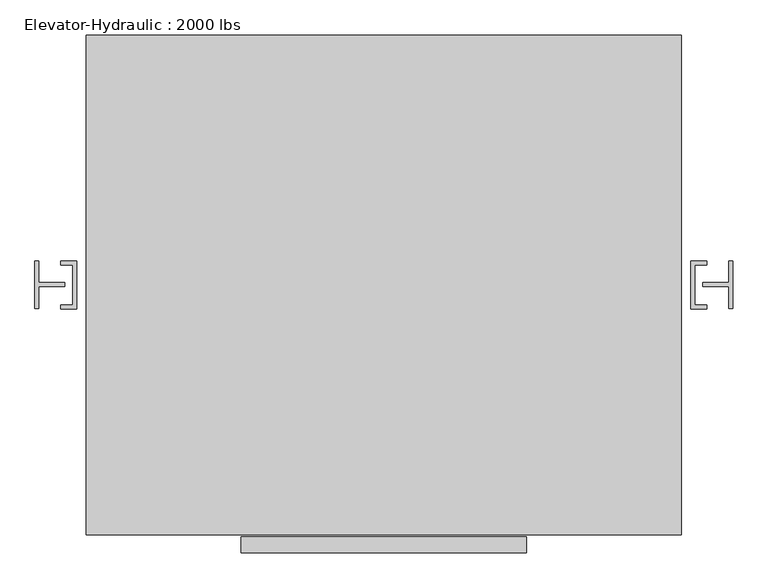
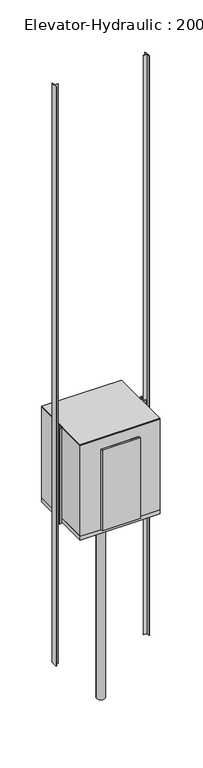
"""IFC4 building model written with IfcOpenShell, lengths in millimetres: proxy geometry, Elevator-Hydraulic : 2000 lbs."""

from ifc_helpers import new_model, si_unit, point, frame, frame_2d, origin, origin_with_axes, place, context, project, spatial, polyline, circle_curve, trimmed, segment, composite_curve, outline, extrude, faceted_brep, source, transform, mapped, element, save


def elevator_hydraulic_2000_lbs_23fd6a1c(model_context):
    return source(origin(), model_context, "Body", "SolidModel", [
        faceted_brep([(-945.0530035, -797.2781737, 5943.6), (959.9469965, -797.2781737, 5943.6), (959.9469965, 802.9218263, 5943.6), (-945.0530035, 802.9218263, 5943.6), (921.8469965, 764.8218263, 5943.6), (921.8469965, -759.1781737, 5943.6), (-906.9530035, -759.1781737, 5943.6), (-906.9530035, 764.8218263, 5943.6), (-906.9530035, 764.8218263, 3657.6), (-906.9530035, -759.1781737, 3657.6), (-449.7530035, -759.1781737, 3657.6), (-449.7530035, -797.2781737, 3657.6), (-945.0530035, -797.2781737, 3657.6), (-945.0530035, 802.9218263, 3657.6), (959.9469965, 802.9218263, 3657.6), (959.9469965, -797.2781737, 3657.6), (464.6469965, -797.2781737, 3657.6), (464.6469965, -759.1781737, 3657.6), (921.8469965, -759.1781737, 3657.6), (921.8469965, 764.8218263, 3657.6), (464.6469965, 764.8218263, 3657.6), (-449.7530035, 764.8218263, 3657.6), (464.6469965, -759.1781737, 5689.6), (-449.7530035, -759.1781737, 5689.6), (-449.7530035, -797.2781737, 5689.6), (464.6469965, -797.2781737, 5689.6)], [[[0, 1, 2, 3], [4, 5, 6, 7]], [[8, 9, 10, 11, 12, 13, 14, 15, 16, 17, 18, 19, 20, 21]], [[5, 4, 19, 18]], [[6, 5, 18, 17, 22, 23, 10, 9]], [[7, 6, 9, 8]], [[4, 7, 8, 21, 20, 19]], [[1, 0, 12, 11, 24, 25, 16, 15]], [[2, 1, 15, 14]], [[3, 2, 14, 13]], [[0, 3, 13, 12]], [[22, 25, 24, 23]], [[23, 24, 11, 10]], [[25, 22, 17, 16]]]),
        extrude(outline(polyline([(464.6469965, -803.6281737), (464.6469965, -854.4281737), (-449.7530035, -854.4281737), (-449.7530035, -803.6281737), (464.6469965, -803.6281737)])), frame((0.0, 0.0, 3657.6), z_axis=(0.0, 0.0, 1.0), x_axis=(1.0, 0.0, 0.0)), (0.0, 0.0, 1.0), 2032.0),
        extrude(outline(polyline([(959.9469965, 802.9218263), (959.9469965, -797.2781737), (-945.0530035, -797.2781737), (-945.0530035, 802.9218263), (959.9469965, 802.9218263)])), frame((0.0, 0.0, 5943.6), z_axis=(0.0, 0.0, 1.0), x_axis=(1.0, 0.0, 0.0)), (0.0, 0.0, 1.0), 25.4),
        extrude(outline(composite_curve([segment(trimmed(circle_curve(frame_2d((7.4469965, 2.8218263)), 101.6), [point((-94.1530035, 2.8218263))], [point((109.0469965, 2.8218263))], False, "CARTESIAN"), True, "CONTINUOUS"), segment(trimmed(circle_curve(frame_2d((7.4469965, 2.8218263)), 101.6), [point((109.0469965, 2.8218263))], [point((-94.1530035, 2.8218263))], False, "CARTESIAN"), True, "CONTINUOUS")], self_intersect=False)), frame((0.0, 0.0, -1219.2), z_axis=(0.0, 0.0, 1.0), x_axis=(1.0, 0.0, 0.0)), (0.0, 0.0, 1.0), 4775.2),
        extrude(outline(polyline([(959.9469965, 802.9218263), (959.9469965, -797.2781737), (-945.0530035, -797.2781737), (-945.0530035, 802.9218263), (959.9469965, 802.9218263)])), frame((0.0, 0.0, 3556.0), z_axis=(0.0, 0.0, 1.0), x_axis=(1.0, 0.0, 0.0)), (0.0, 0.0, 1.0), 101.6),
        extrude(outline(polyline([(-976.8030035, 79.0218263), (-976.8030035, -73.3781737), (-1027.6030035, -73.3781737), (-1027.6030035, -60.6781737), (-989.5030035, -60.6781737), (-989.5030035, 66.3218263), (-1027.6030035, 66.3218263), (-1027.6030035, 79.0218263), (-976.8030035, 79.0218263)])), frame((0.0, 0.0, 3556.0), z_axis=(0.0, 0.0, 1.0), x_axis=(1.0, 0.0, 0.0)), (0.0, 0.0, 1.0), 2413.0),
        extrude(outline(polyline([(991.6969965, 79.0218263), (1042.4969965, 79.0218263), (1042.4969965, 66.3218263), (1004.3969965, 66.3218263), (1004.3969965, -60.6781737), (1042.4969965, -60.6781737), (1042.4969965, -73.3781737), (991.6969965, -73.3781737), (991.6969965, 79.0218263)])), frame((0.0, 0.0, 3556.0), z_axis=(0.0, 0.0, 1.0), x_axis=(1.0, 0.0, 0.0)), (0.0, 0.0, 1.0), 2413.0),
        extrude(outline(polyline([(-1097.4530035, 79.0218263), (-1097.4530035, 9.1718263), (-1014.9030035, 9.1718263), (-1014.9030035, -3.5281737), (-1097.4530035, -3.5281737), (-1097.4530035, -73.3781737), (-1110.1530035, -73.3781737), (-1110.1530035, 79.0218263), (-1097.4530035, 79.0218263)])), origin_with_axes(), (0.0, 0.0, 1.0), 14630.4),
        extrude(outline(polyline([(1112.3469965, 79.0218263), (1125.0469965, 79.0218263), (1125.0469965, -73.3781737), (1112.3469965, -73.3781737), (1112.3469965, -3.5281737), (1029.7969965, -3.5281737), (1029.7969965, 9.1718263), (1112.3469965, 9.1718263), (1112.3469965, 79.0218263)])), origin_with_axes(), (0.0, 0.0, 1.0), 14630.4),
    ])


if __name__ == "__main__":
    model = new_model("IFC4")
    model_context = context("Model", 3, world=origin())
    ifc_project = project(units=[si_unit("LENGTHUNIT", "METRE", prefix="MILLI")], contexts=[model_context])
    site = spatial("IfcSite", under=ifc_project)
    building = spatial("IfcBuilding", under=site)
    placement = place(None, origin())
    elevator_hydraulic_2000_lbs_shape = elevator_hydraulic_2000_lbs_23fd6a1c(model_context)
    element("IfcBuildingElementProxy", 1, Name="Elevator-Hydraulic : 2000 lbs", ObjectType="Elevator-Hydraulic : 2000 lbs", at=placement, inside=building, context=model_context, shape_type="MappedRepresentation", body=[
        mapped(elevator_hydraulic_2000_lbs_shape, transform((0.0, 0.0, 0.0), x_axis=(1.0, 0.0, 0.0), y_axis=(0.0, 1.0, 0.0), z_axis=(0.0, 0.0, 1.0))),
    ])
    save(model, "model.ifc")

# Revit data of these elements
# Type "Elevator-Hydraulic : 2000 lbs"
#   Cab Location = 12' - 0"
#   Width = 7' - 4"
#   Pit Depth = 4' - 0"
#   Height [instance default] = 36' - 0"
#   Door Opening = 3' - 0"
#   Depth = 5' - 9"
#   Cab Width = 6' - 0"
#   Cab Height = 7' - 6"
#   Cab Depth = 5' - 0"
#   Default Elevation = 0
# Element 1 (IfcBuildingElementProxy, "Elevator-Hydraulic : 2000 lbs")
#   Height = 48' - 0"
#   Materials on its faces: "Metal - Steel"
# Materials
#   "Metal - Steel": class "Metal", colour RGB 247 247 247, transparency 0
